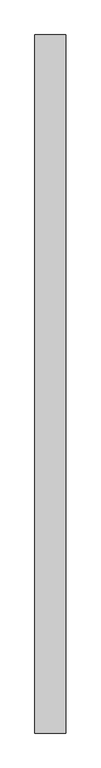
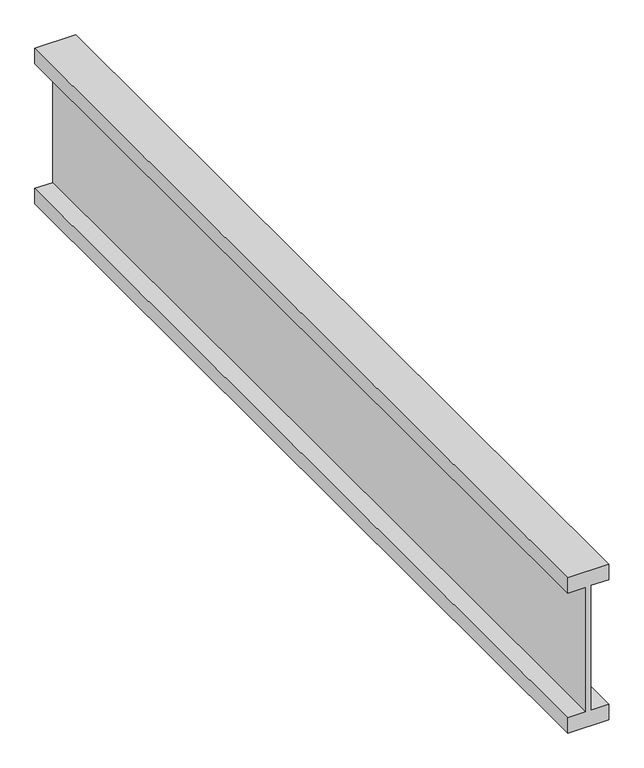
"""IFC4 building model written with IfcOpenShell, lengths in millimetres: proxy geometry, Framing18:Framing065:302447 : Framing18:Framing065:302447."""

from ifc_helpers import new_model, si_unit, frame, origin, place, context, project, spatial, polyline, outline, extrude, source, transform, mapped, element, save


def generic_models_92f52601(model_context):
    return source(origin(), model_context, "Body", "SweptSolid", [
        extrude(outline(polyline([(40077.771, 12834.411296), (40077.771, 12873.305046), (39792.021, 12873.305046), (39792.021, 12834.411296), (39757.096, 12834.411296), (39757.096, 12923.311296), (39792.021, 12923.311296), (39792.021, 12884.417546), (40077.771, 12884.417546), (40077.771, 12923.311296), (40112.696, 12923.311296), (40112.696, 12834.411296), (40077.771, 12834.411296)])), frame((0.0, -3469.6166527, 0.0), z_axis=(0.0, 1.0, 0.0), x_axis=(0.0, 0.0, 1.0)), (0.0, 0.0, 1.0), 2000.0),
    ])


if __name__ == "__main__":
    model = new_model("IFC4")
    model_context = context("Model", 3, world=origin())
    ifc_project = project(units=[si_unit("LENGTHUNIT", "METRE", prefix="MILLI")], contexts=[model_context])
    site = spatial("IfcSite", under=ifc_project)
    building = spatial("IfcBuilding", under=site)
    placement = place(None, origin())
    generic_models_shape = generic_models_92f52601(model_context)
    element("IfcBuildingElementProxy", 1, Name="Framing18:Framing065:302447 : Framing18:Framing065:302447", ObjectType="Framing18:Framing065:302447 : Framing18:Framing065:302447", at=placement, inside=building, context=model_context, shape_type="MappedRepresentation", body=[
        mapped(generic_models_shape, transform((0.0, 0.0, 0.0), x_axis=(1.0, 0.0, 0.0), y_axis=(0.0, 1.0, 0.0), z_axis=(0.0, 0.0, 1.0))),
    ])
    save(model, "model.ifc")

# Revit data of these elements
# Type "Framing18:Framing065:302447 : Framing18:Framing065:302447"
#   NameOverride = "Framing18:Framing065:302447"
#   ObjectTypeOverride = "Framing18:Framing065"
#   Reference = "Framing065"
#   Category = "Generic Models"
#   Tag = "302447"
# Element 1 (IfcBuildingElementProxy, "Framing18:Framing065:302447 : Framing18:Framing065:302447")
#   Materials on its faces: "WOOD FRAMING (SEE STRUCT DWGS)"
# Materials
#   "WOOD FRAMING (SEE STRUCT DWGS)": class "Unassigned", colour RGB 224 188 168, transparency 0, Cost = 0
